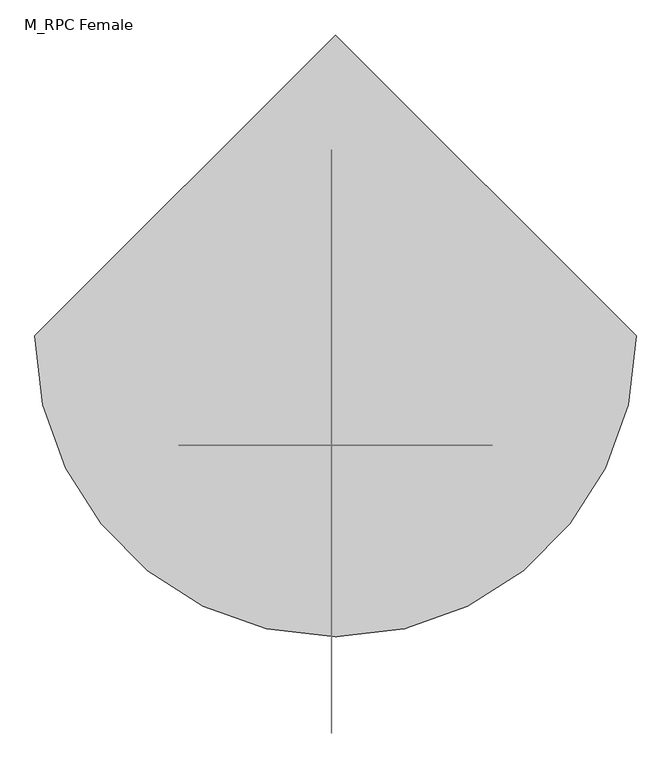
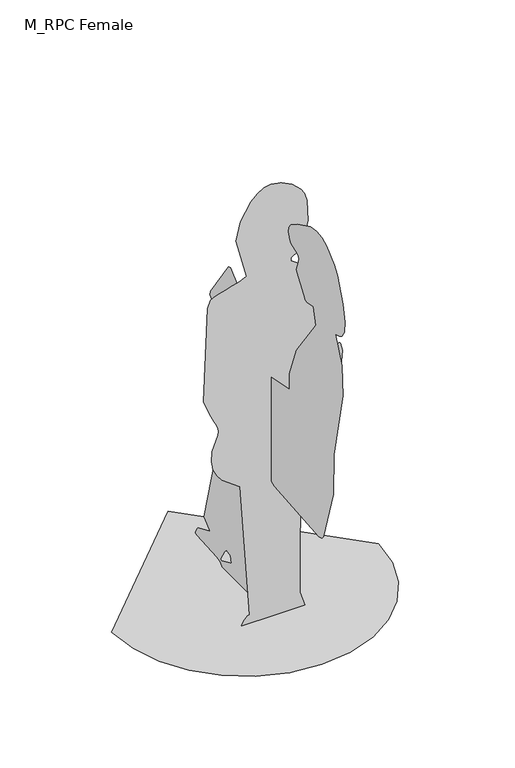
"""IFC4 building model written with IfcOpenShell, lengths in millimetres: proxy geometry, M_RPC Female : Cynthia."""

from ifc_helpers import new_model, si_unit, origin, place, context, project, spatial, triangles, source, transform, mapped, element, save


def m_rpc_female_e5f04239(model_context):
    return source(origin(), model_context, "Body", "Tessellation", [
        triangles([(-437.3057565, 0.0, 2.93e-05), (-425.7448342, -100.2015691, 2.93e-05), (-392.8194094, -192.2206799, 2.93e-05), (-341.1658762, -273.4208834, 2.93e-05), (-273.4209015, -341.1659489, 2.93e-05), (-192.2206254, -392.819373, 2.93e-05), (-100.2015237, -425.7447979, 2.93e-05), (1.91e-05, -437.3057565, 2.93e-05), (100.2015782, -425.7448342, 2.93e-05), (192.220698, -392.8194094, 2.93e-05), (273.4209015, -341.1658762, 2.93e-05), (341.1660215, -273.4209015, 2.93e-05), (392.819373, -192.2206072, 2.93e-05), (425.7447979, -100.2014965, 2.93e-05), (437.3057565, 3.36e-05, 2.93e-05), (-5.73e-05, 437.3057928, 2.93e-05), (-5.5814555, 72.246871, 69.496344), (-5.5814561, 67.031142, 46.0256608), (-5.5814583, 124.4039254, 19.9471336), (-5.5814583, 129.6196318, 25.1628196), (-5.5814566, 107.6002273, 62.2269385), (-5.5814561, 95.7175496, 74.7120321), (-5.5814561, -28.6037069, 4.4e-06), (-5.5814555, -39.8908654, 35.5942482), (-5.5814555, -42.4985551, 37.2668205), (-5.5814544, -45.6385706, 39.1828009), (-5.5814544, -48.9915363, 41.1595652), (-5.5814544, -52.2381223, 43.0148345), (-5.5814544, -55.0589122, 44.56573), (-5.5814544, -57.1346076, 45.6302408), (-5.5814544, -58.1458059, 46.0256654), (-5.5814555, -58.1458876, 5.3e-06), (-5.5814555, -108.9534241, 6.8e-06), (-5.5814544, -116.5758149, 29.8220214), (-5.5814504, -109.3236867, 163.616957), (-5.5814413, -45.457159, 488.7457126), (-5.5814407, -47.714434, 510.223653), (-5.5814407, -52.9301222, 512.8314517), (-5.5814407, -176.6935208, 461.1352976), (-5.5814373, -431.0100652, 441.4516517), (-5.5814373, -446.7160832, 445.0273055), (-5.5814368, -456.1585665, 455.8251566), (-5.58143, -511.6809405, 636.0529638), (-5.581426, -514.5203021, 776.2247131), (-5.5814186, -566.7671494, 1012.4528812), (-5.5814158, -561.4616592, 1112.6378271), (-5.5814129, -522.3438071, 1198.6970364), (-5.5814129, -544.7658397, 1204.5966036), (-5.5814118, -561.2097487, 1214.9815075), (-5.5814118, -573.9143148, 1236.2570984), (-5.5814101, -577.4586843, 1272.8740494), (-5.5814084, -566.4219306, 1329.2825249), (-5.5814067, -535.3830912, 1409.9332706), (-5.5814067, -516.7872059, 1433.7636475), (-5.5814055, -472.5754423, 1474.3204742), (-5.5814055, -445.9832065, 1486.7813416), (-5.5814067, -415.7490417, 1491.1880493), (-5.5814067, -381.3846422, 1485.4068615), (-5.5814084, -308.1102631, 1450.1703495), (-5.5814101, -271.6907746, 1426.3735462), (-5.5814107, -259.9822778, 1410.5514015), (-5.5814118, -256.5008769, 1391.3528641), (-5.5814118, -264.1662884, 1368.2074745), (-5.5814118, -270.5525991, 1361.5164585), (-5.5814118, -307.4893707, 1345.9730759), (-5.5814118, -313.6895373, 1341.0963387), (-5.5814118, -316.3233519, 1334.3053288), (-5.5814129, -314.5104538, 1321.5896805), (-5.5814141, -303.2841405, 1289.971843), (-5.5814141, -303.9328654, 1281.3184467), (-5.5814146, -344.8551496, 1227.4567635), (-5.5814158, -350.2254976, 1216.9519541), (-5.5814158, -354.0100413, 1213.137216), (-5.5814158, -360.9104559, 1211.8311184), (-5.5814146, -397.1668911, 1216.9519541), (-5.5814158, -412.8139375, 1162.1870556), (-5.581422, -300.7217424, 1007.464959), (-5.581426, -262.9222146, 903.7019611), (-5.5814277, -261.5584715, 849.2446747), (-5.58143, -151.2454102, 828.1022152), (-5.58143, -131.1657765, 828.3817766), (-5.5814288, -146.9133073, 873.4847649), (-5.5814288, -146.8129046, 875.3230974), (-5.5814288, -136.5283852, 880.5989382), (-5.581426, 66.2908528, 1062.7618744), (-5.581426, 72.9541861, 1068.1172161), (-5.5814266, 85.3175848, 1063.7719145), (-5.5814322, 186.9119923, 916.7356859), (-5.5814328, 189.6002729, 904.0095005), (-5.5814339, 74.8547106, 802.3032812), (-5.5814345, 53.5231683, 768.5290346), (-5.5814345, 40.9526102, 757.9697954), (-5.5814345, 7.0502408, 750.1462177), (-5.5814362, -30.7395663, 681.3427139), (-5.5814362, -32.0672787, 677.1262562), (-5.5814368, -2.7970168, 673.1418337), (-5.5814379, 74.8547106, 666.6947708), (-5.5814566, 223.5023279, 113.8298615), (-5.5814572, 192.3027606, 86.4272282), (-5.5814572, 189.6002729, 82.5355962), (-5.5814595, 257.4045281, 53.849234), (-5.5814595, 261.0572667, 50.6335418), (-5.5814595, 266.9932234, 41.9573409), (-5.58146, 270.4022813, 33.1798288), (-5.58146, 270.8965462, 29.8373185), (-5.58146, 270.443685, 27.7706614), (-5.58146, 262.21192, 24.6723971), (-5.5814583, 148.3989361, 17.7234776), (-5.5814583, 129.6196318, 12.1235594), (-5.5814583, 119.2279423, 0.0), (-103.2161017, -158.8625416, 3.138314), (-93.5649194, -158.8625416, 19.242982), (-88.6211895, -158.8625416, 24.4594286), (-82.9717796, -158.8625416, 28.4095146), (-76.7113605, -158.8625416, 30.3784918), (-108.0056168, -158.8625779, 484.1449396), (-166.5178156, -158.8625779, 527.9969504), (-183.6322324, -158.8625779, 549.73316), (-196.1559229, -158.8625779, 575.232294), (-202.0512208, -158.8625779, 604.6166196), (-199.2805142, -158.8625779, 638.0082951), (-180.7337175, -158.8625779, 688.9249546), (-179.5104455, -158.8625779, 700.1737593), (-181.025542, -158.8625779, 711.0281839), (-186.0298695, -158.8625779, 724.8027792), (-192.7431225, -158.8625779, 739.7135696), (-208.5562016, -158.8625779, 771.7149593), (-227.9668809, -158.8625779, 820.5580536), (-215.5926726, -158.8626143, 1139.7189503), (-204.4961842, -158.8626143, 1164.7947453), (-195.70417, -158.8626143, 1170.2244284), (-178.399812, -158.8626143, 1176.5899555), (-156.0960135, -158.8626143, 1183.4364126), (-132.3055416, -158.8626143, 1190.3077229), (-110.5413086, -158.8626143, 1196.7492628), (-94.3160908, -158.8626143, 1202.3054644), (-87.1427823, -158.8626143, 1206.520396), (-121.0448735, -158.8626143, 1339.5209988), (-105.9598205, -158.8626324, 1402.4766037), (-72.2006347, -158.8626324, 1459.392897), (-51.1398926, -158.8626324, 1480.6086079), (-28.7965572, -158.8626324, 1494.3413452), (-6.2993123, -158.8626324, 1498.5999516), (28.3785935, -158.8626324, 1491.3003971), (62.9443729, -158.8626324, 1473.3395748), (92.2084342, -158.8626324, 1445.5309525), (103.2305721, -158.8626324, 1428.1879704), (112.1216355, -158.8626324, 1400.9896305), (114.2135136, -158.8626143, 1329.2264236), (96.1614451, -158.8626143, 1258.9092041), (79.8725593, -158.8626143, 1233.5183121), (58.89705, -158.8626143, 1219.5597164), (58.89705, -158.8626143, 1209.128231), (105.4402574, -158.8626143, 1177.1569994), (186.6818646, -158.8626143, 1146.5396822), (190.9101676, -158.8626143, 1130.2527403), (197.4604945, -158.8625961, 874.5614433), (217.1152177, -158.8625961, 870.6124111), (219.4354431, -158.8625961, 869.5266489), (221.3548754, -158.8625961, 866.986179), (227.9668991, -158.8625779, 839.7665468), (217.9761209, -158.8625779, 726.675412), (216.778683, -158.8625779, 725.536964), (198.418848, -158.8625779, 721.3532078), (197.1132955, -158.8625779, 721.4596693), (188.2934486, -158.8625779, 736.0850121), (176.2504519, -158.8625779, 750.1460724), (172.5434834, -158.8625779, 744.3784012), (169.4576071, -158.8625779, 737.6237263), (166.7654749, -158.8625779, 730.2867468), (164.2397206, -158.8625779, 722.7717985), (161.6530689, -158.8625779, 715.4834352), (158.7781536, -158.8625779, 708.8262835), (155.3876265, -158.8625779, 703.2046789), (164.598783, -158.8625779, 582.3864721), (159.7288041, -158.8625779, 557.993666), (150.1719383, -158.8625779, 536.3020758), (143.4521541, -158.8625779, 528.6086137), (105.433708, -158.8625779, 509.5447337), (96.8765541, -158.8625779, 503.2554737), (90.1912608, -158.8625779, 494.5763523), (88.7455914, -158.8625416, 49.4103652), (105.4366057, -158.8625416, 7.4e-05), (-104.3910027, -158.8625416, 7.4e-05)], [[15, 16, 1], [14, 15, 1], [14, 1, 2], [13, 14, 2], [13, 2, 3], [13, 3, 4], [12, 13, 4], [11, 12, 4], [11, 4, 5], [11, 5, 6], [11, 6, 7], [11, 7, 8], [11, 8, 9], [11, 9, 10], [23, 17, 18], [110, 23, 18], [110, 18, 19], [109, 110, 19], [17, 23, 24], [31, 32, 33], [31, 33, 34], [109, 19, 20], [108, 109, 20], [88, 89, 90], [82, 83, 84], [85, 86, 87], [105, 106, 107], [104, 105, 107], [103, 104, 107], [102, 103, 107], [101, 102, 107], [100, 101, 107], [100, 107, 108], [100, 108, 20], [100, 20, 21], [100, 21, 22], [87, 88, 90], [85, 87, 90], [84, 85, 90], [84, 90, 91], [84, 91, 92], [84, 92, 93], [82, 84, 93], [81, 82, 93], [81, 93, 94], [80, 81, 94], [80, 94, 95], [99, 100, 22], [17, 24, 25], [17, 25, 26], [31, 34, 35], [30, 31, 35], [17, 26, 27], [17, 27, 28], [17, 28, 29], [29, 30, 35], [17, 29, 35], [22, 17, 35], [99, 22, 35], [98, 99, 35], [97, 98, 35], [97, 35, 36], [97, 36, 37], [96, 97, 37], [96, 37, 38], [95, 96, 38], [80, 95, 38], [80, 38, 39], [79, 80, 39], [79, 39, 40], [79, 40, 41], [79, 41, 42], [79, 42, 43], [79, 43, 44], [78, 79, 44], [77, 78, 44], [77, 44, 45], [77, 45, 46], [76, 77, 46], [76, 46, 47], [75, 76, 47], [72, 73, 74], [71, 72, 74], [61, 62, 63], [60, 61, 63], [60, 63, 64], [59, 60, 64], [59, 64, 65], [59, 65, 66], [58, 59, 66], [57, 58, 66], [56, 57, 66], [55, 56, 66], [54, 55, 66], [54, 66, 67], [53, 54, 67], [52, 53, 67], [52, 67, 68], [51, 52, 68], [50, 51, 68], [49, 50, 68], [48, 49, 68], [47, 48, 68], [75, 47, 68], [74, 75, 68], [71, 74, 68], [70, 71, 68], [69, 70, 68], [183, 184, 111], [183, 111, 112], [183, 112, 113], [183, 113, 114], [183, 114, 115], [182, 183, 115], [181, 182, 115], [181, 115, 116], [154, 155, 156], [164, 165, 166], [180, 181, 116], [163, 164, 166], [162, 163, 166], [162, 166, 167], [161, 162, 167], [160, 161, 167], [159, 160, 167], [158, 159, 167], [157, 158, 167], [180, 116, 117], [180, 117, 118], [180, 118, 119], [180, 119, 120], [180, 120, 121], [180, 121, 122], [179, 180, 122], [179, 122, 123], [178, 179, 123], [177, 178, 123], [176, 177, 123], [175, 176, 123], [174, 175, 123], [174, 123, 124], [174, 124, 125], [173, 174, 125], [172, 173, 125], [171, 172, 125], [170, 171, 125], [169, 170, 125], [169, 125, 126], [168, 169, 126], [168, 126, 127], [167, 168, 127], [157, 167, 127], [157, 127, 128], [156, 157, 128], [154, 156, 128], [153, 154, 128], [153, 128, 129], [153, 129, 130], [153, 130, 131], [153, 131, 132], [153, 132, 133], [153, 133, 134], [153, 134, 135], [153, 135, 136], [153, 136, 137], [152, 153, 137], [151, 152, 137], [150, 151, 137], [149, 150, 137], [149, 137, 138], [149, 138, 139], [148, 149, 139], [147, 148, 139], [146, 147, 139], [146, 139, 140], [145, 146, 140], [145, 140, 141], [144, 145, 141], [144, 141, 142], [144, 142, 143]], closed=False),
    ])


if __name__ == "__main__":
    model = new_model("IFC4")
    model_context = context("Model", 3, world=origin())
    ifc_project = project(units=[si_unit("LENGTHUNIT", "METRE", prefix="MILLI")], contexts=[model_context])
    site = spatial("IfcSite", under=ifc_project)
    building = spatial("IfcBuilding", under=site)
    placement = place(None, origin())
    m_rpc_female_shape = m_rpc_female_e5f04239(model_context)
    element("IfcBuildingElementProxy", 1, Name="M_RPC Female : Cynthia", ObjectType="M_RPC Female : Cynthia", at=placement, inside=building, context=model_context, shape_type="MappedRepresentation", body=[
        mapped(m_rpc_female_shape, transform((0.0, 0.0, 0.0), x_axis=(1.0, 0.0, 0.0), y_axis=(0.0, 1.0, 0.0), z_axis=(0.0, 0.0, 1.0))),
    ])
    save(model, "model.ifc")

# Revit data of these elements
# Type "M_RPC Female : Cynthia"
#   built-in parameter 1005198 = "{2, 15},{22, RPC-8-FXA2-QQQ0-UGV2-6},{1, 0},{1, 0},{2, 37},{1, 8},{5, Color},{1, 0},{1, 0},{3, 0.8},{3, 0.8},{3, 0.8},{1, 8},{7, BBoxMin},{1, 0},{1, 0},{1, 0},{1, 0},{1, 0},{1, 8},{7, BBoxMax},{1, 0},{1, 0},{1, 0},{1, 0},{1, 0},{2, 11},{9, RPCTypeId},{1, 0},{1, 0},{22, RPC-8-FXA2-QQQ0-UGV2-6},{1, 6},{14, RPCPlantHeight},{1, 0},{1, 0},{7, 4.91667},{2, 11},{7, keyword},{1, 0},{1, 0},{117, :Geometry:RPC:Cynthia:seated:casual:female:caucasian:black pants:black shoes:black jacket:looking through file folder},{2, 11},{8, category},{1, 0},{1, 0},{25, :People [Seated-Business]},{2, 11},{12, LocalizedUID},{1, 0},{1, 0},{7, Cynthia},{2, 14},{6, Height},{1, 0},{1, 0},{7, 4.91667},{1, 2},{16, Cast Reflections},{1, 0},{1, 0},{1, 0},{1, 2},{6, Jitter},{1, 0},{1, 0},{1, 1},{1, 2},{9, Billboard},{1, 0},{1, 0},{1, 0},{1, 2},{12, Cast Shadows},{1, 0},{1, 0},{1, 1},{1, 2},{20, Apply Filter Effects},{1, 0},{1, 0},{1, 0},{2, 11},{28, Apply Filter Effects-Text-FC},{1, 0},{1, 0},{4, None},{2, 11},{20, AdvancedUIDefinition},{1, 0},{1, 0},{0, },{2, 11},{10, AssetLibID},{1, 0},{1, 0},{36, 4D3F6E72-3F99-4203-98E9-AF80B3C7A7A4},{2, 11},{10, BaseSchema},{1, 0},{1, 0},{9, RPCSchema},{2, 11},{12, ExchangeGUID},{1, 0},{1, 0},{0, },{1, 2},{6, Hidden},{1, 0},{1, 0},{1, 0},{1, 4},{11, RPCCategory},{1, 0},{1, 0},{1, 0},{2, 11},{8, RPCImage},{1, 0},{1, 0},{0, },{1, 4},{13, SchemaVersion},{1, 0},{1, 0},{1, 4},{2, 11},{12, UIDefinition},{1, 0},{1, 0},{0, },{2, 11},{6, UIName},{1, 0},{1, 0},{22, RPC-8-FXA2-QQQ0-UGV2-6},{2, 11},{11, VersionGUID},{1, 0},{1, 0},{9, RPCSchema},{2, 11},{9, assettype},{1, 0},{1, 0},{11, RPCGeometry},{2, 11},{11, description},{1, 0},{1, 0},{0, },{2, 11},{9, localname},{1, 0},{1, 0},{3, RPC},{2, 11},{9, localtype},{1, 0},{1, 0},{3, RPC},{1, 4},{8, revision},{1, 0},{1, 0},{1, 1},{2, 11},{9, thumbnail},{1, 0},{1, 0},{0, },{1, 4},{7, version},{1, 0},{1, 0},{1, 1},{1, 2},{20, RPC_Cast Reflections},{1, 0},{1, 0},{1, 1},{1, 2},{10, RPC_Jitter},{1, 0},{1, 0},{1, 1},{1, 2},{13, RPC_Billboard},{1, 0},{1, 0},{1, 0},{1, 2},{16, RPC_Cast Shadows},{1, 0},{1, 0},{1, 1},{21, assetlibrary_base.fbx},{1, 5},"
#   built-in parameter 1005195 = "RPC-8-FXA2-QQQ0-UGV2-6"
#   Height = 0
